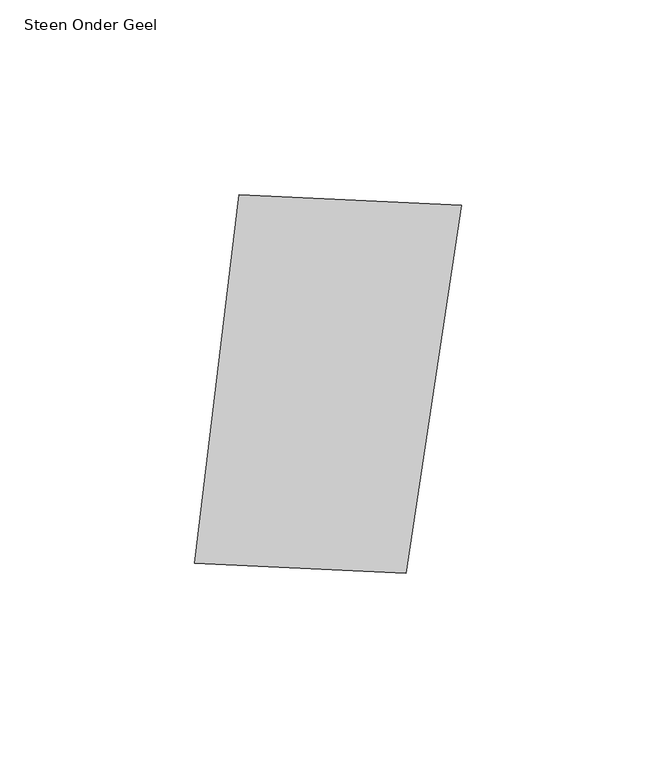
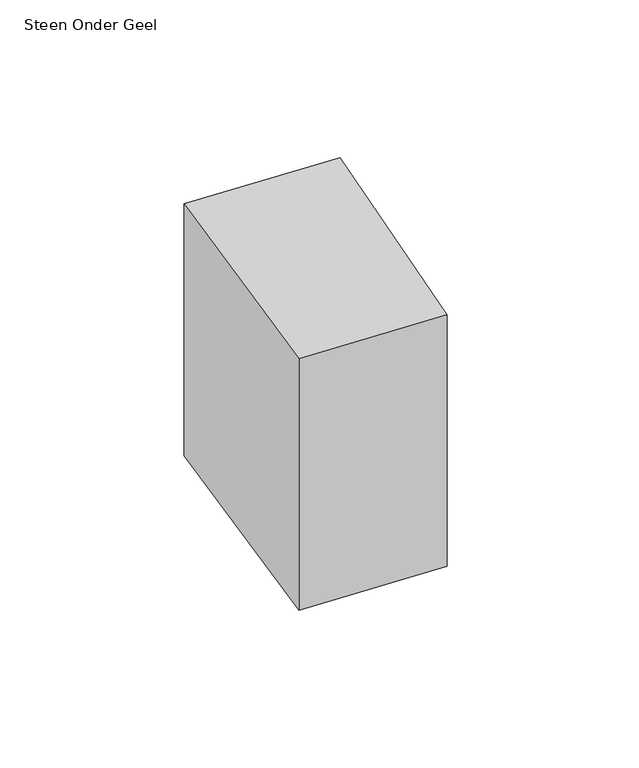
"""IFC4 building model written with IfcOpenShell, lengths in millimetres: proxy geometry, 00_GMA_steen_versie_4 : Steen Onder Geel."""

from ifc_helpers import new_model, si_unit, origin, origin_with_axes, place, context, project, spatial, polyline, outline, extrude, source, transform, mapped, element, save


def steen_onder_geel_94529cec(model_context):
    return source(origin(), model_context, "Body", "SweptSolid", [
        extrude(outline(polyline([(107.3151447, 113.588548), (93.0561577, 19.1377634), (38.8107085, 21.7371267), (50.2937565, 116.3101398), (107.3151447, 113.588548)])), origin_with_axes(), (0.0, 0.0, 1.0), 100.0),
    ])


if __name__ == "__main__":
    model = new_model("IFC4")
    model_context = context("Model", 3, world=origin())
    ifc_project = project(units=[si_unit("LENGTHUNIT", "METRE", prefix="MILLI")], contexts=[model_context])
    site = spatial("IfcSite", under=ifc_project)
    building = spatial("IfcBuilding", under=site)
    placement = place(None, origin())
    steen_onder_geel_shape = steen_onder_geel_94529cec(model_context)
    element("IfcBuildingElementProxy", 1, Name="00_GMA_steen_versie_4 : Steen Onder Geel", ObjectType="00_GMA_steen_versie_4 : Steen Onder Geel", at=placement, inside=building, context=model_context, shape_type="MappedRepresentation", body=[
        mapped(steen_onder_geel_shape, transform((0.0, 0.0, 0.0), x_axis=(1.0, 0.0, 0.0), y_axis=(0.0, 1.0, 0.0), z_axis=(0.0, 0.0, 1.0))),
    ])
    save(model, "model.ifc")

# Revit data of these elements
# Type "00_GMA_steen_versie_4 : Steen Onder Geel"
#   StootVoegHalfBoven [instance default] = 5 mm
#   StootVoegHalf [instance default] = 5 mm
#   StootVoegBreedteOnder = 10 mm
#   StootVoegBreedteBoven = 10 mm
#   Steendikte = 100 mm
#   LintVoegOnderHalf = 0 mm
#   LintVoegOnder = 0 mm
#   LintVoegBovenHalf = 5 mm
#   LintVoegBoven = 10 mm
#   materiaal = 21_steen_geel
#   MateriaalVoeg = none
#   Default Elevation = 0
# Element 1 (IfcBuildingElementProxy, "00_GMA_steen_versie_4 : Steen Onder Geel")
#   Materials on its faces: "21_steen_geel"
# Materials
#   "21_steen_geel": class "Unassigned", colour RGB 202 202 0, transparency 0, Cost = 0
